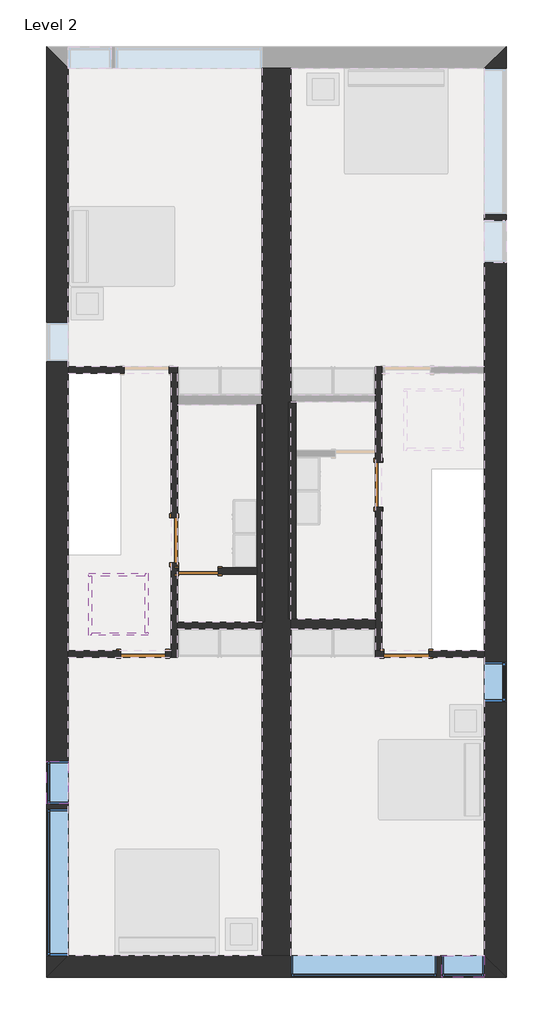
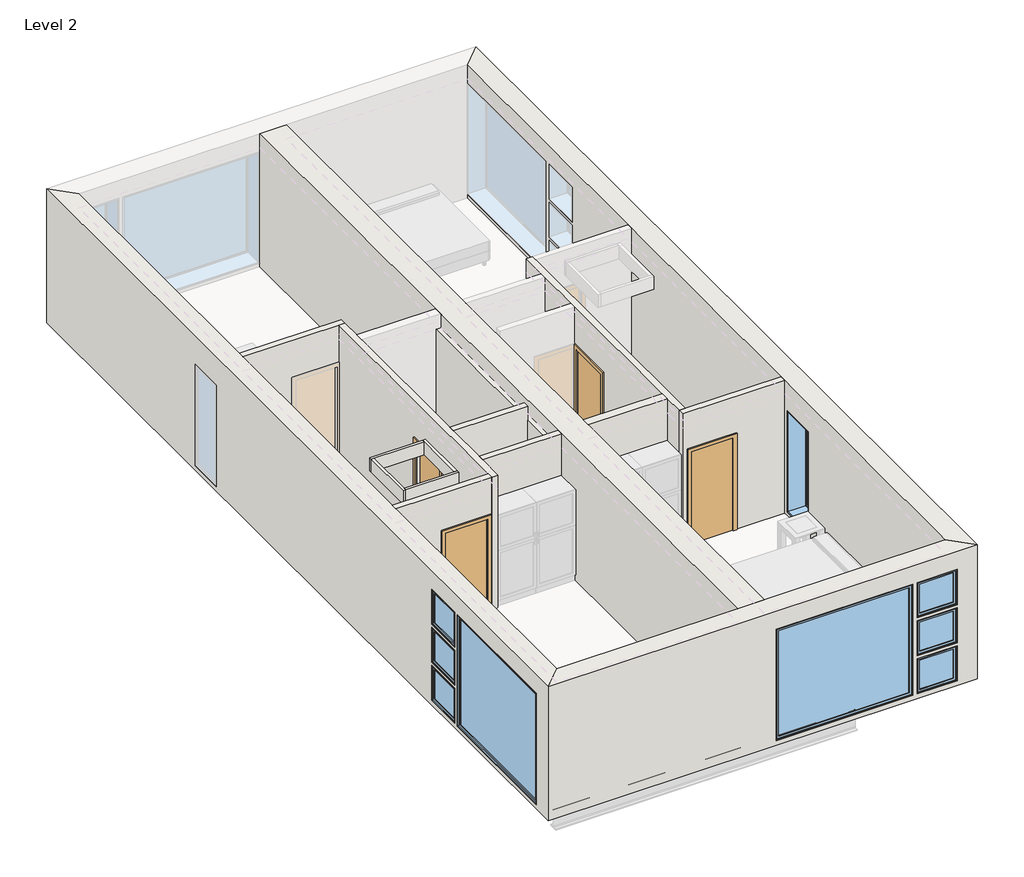
# One storey, part 1 of 2: 20 walls, 9 windows, 5 doors.
"""IFC4 building model written with IfcOpenShell, lengths in millimetres."""

import ifcopenshell
import ifcopenshell.guid

model = None  # the IFC model being written
_history = None  # IfcOwnerHistory: only IFC2X3 demands one
_inside = {}  # id of a spatial element -> (the spatial element, [elements in it])
_under = {}  # id of a project, library or spatial element -> (it, [spatial elements below it])
_declared = {}  # id of a project -> (the project, [libraries it declares])
_typed = {}  # id of a type object -> (the type object, [elements of that type])
_made_of = {}  # id of a material, layer set ... -> (it, [elements and type objects made of it])


def new_model(schema):
    """Start an empty IFC model of exactly this schema.

    Asked for "IFC4X3", IfcOpenShell would pick the latest addendum, in which some entities
    have other attributes; the version numbers below select the first issue.
    IFC2X3 requires an IfcOwnerHistory on every rooted entity: one is made here for all.
    """
    global model, _history
    if schema == "IFC4X3":
        model = ifcopenshell.file(schema_version=(4, 3, 0, 0))
    else:
        model = ifcopenshell.file(schema=schema)
    _inside.clear()
    _under.clear()
    _declared.clear()
    _typed.clear()
    _made_of.clear()
    _history = None
    if model.schema == "IFC2X3":
        org = make("IfcOrganization", Name="unknown")
        user = make(
            "IfcPersonAndOrganization",
            ThePerson=make("IfcPerson", FamilyName="unknown"),
            TheOrganization=org,
        )
        app = make(
            "IfcApplication",
            ApplicationDeveloper=org,
            Version="unknown",
            ApplicationFullName="unknown",
            ApplicationIdentifier="unknown",
        )
        _history = make(
            "IfcOwnerHistory",
            OwningUser=user,
            OwningApplication=app,
            ChangeAction="ADDED",
            CreationDate=0,
        )
    return model


def make(cls, **values):
    """One entity of the class cls with the attributes given. An attribute that is None is left unset."""
    return model.create_entity(
        cls, **{name: value for name, value in values.items() if value is not None}
    )


def rooted(cls, **values):
    """An entity with a GlobalId (a new one), such as an element, a storey or a relation."""
    return make(cls, GlobalId=ifcopenshell.guid.new(), OwnerHistory=_history, **values)


def si_unit(unit_type, name, prefix=None):
    """IfcSIUnit, for example si_unit("LENGTHUNIT", "METRE", prefix="MILLI")."""
    return make("IfcSIUnit", UnitType=unit_type, Prefix=prefix, Name=name)


def assignment(units):
    """IfcUnitAssignment: the units of a project."""
    return None if units is None else make("IfcUnitAssignment", Units=units)


def point(xyz):
    """IfcCartesianPoint."""
    return None if xyz is None else make("IfcCartesianPoint", Coordinates=xyz)


def direction(xyz):
    """IfcDirection."""
    return None if xyz is None else make("IfcDirection", DirectionRatios=xyz)


def frame(location, z_axis=None, x_axis=None):
    """IfcAxis2Placement3D, a coordinate frame: its origin and axes. An axis left out is left unset."""
    return make(
        "IfcAxis2Placement3D",
        Location=point(location),
        Axis=direction(z_axis),
        RefDirection=direction(x_axis),
    )


def origin():
    """The frame at (0, 0, 0) with its axes left unset."""
    return frame((0.0, 0.0, 0.0))


def origin_with_axes():
    """The frame at (0, 0, 0) with the z axis (0, 0, 1) and the x axis (1, 0, 0) written out."""
    return frame((0.0, 0.0, 0.0), z_axis=(0.0, 0.0, 1.0), x_axis=(1.0, 0.0, 0.0))


def place(relative_to, where):
    """IfcLocalPlacement: puts the frame where relative to a parent placement (None: the world)."""
    return make(
        "IfcLocalPlacement", PlacementRelTo=relative_to, RelativePlacement=where
    )


def context(
    kind, dimensions, precision=None, world=None, true_north=None, identifier=None
):
    """IfcGeometricRepresentationContext, for example the 3D "Model" context."""
    return make(
        "IfcGeometricRepresentationContext",
        ContextIdentifier=identifier,
        ContextType=kind,
        CoordinateSpaceDimension=dimensions,
        Precision=precision,
        WorldCoordinateSystem=world,
        TrueNorth=true_north,
    )


def project(units=None, contexts=None):
    """IfcProject with its units and contexts."""
    return rooted(
        "IfcProject",
        Name="project",
        RepresentationContexts=contexts,
        UnitsInContext=assignment(units),
    )


def spatial(cls, under=None, at=None, **own):
    """A site, building, storey or space (cls), placed at a placement, below another one or the project."""
    s = rooted(cls, ObjectPlacement=at, **own)
    if under is not None:
        _under.setdefault(under.id(), (under, []))[1].append(s)
    return s


def polyline(points):
    """IfcPolyline through the points."""
    return make("IfcPolyline", Points=[point(p) for p in points])


def outline(outer, holes=None, kind="AREA"):
    """IfcArbitraryClosedProfileDef: a profile drawn as a closed curve; with holes, ...WithVoids."""
    if holes is None:
        return make("IfcArbitraryClosedProfileDef", ProfileType=kind, OuterCurve=outer)
    return make(
        "IfcArbitraryProfileDefWithVoids",
        ProfileType=kind,
        OuterCurve=outer,
        InnerCurves=holes,
    )


def extrude(swept, where, along, depth):
    """IfcExtrudedAreaSolid: the profile swept, set in the frame where, extruded along a direction by depth."""
    return make(
        "IfcExtrudedAreaSolid",
        SweptArea=swept,
        Position=where,
        ExtrudedDirection=direction(along),
        Depth=depth,
    )


def faces_of(points, faces, orient=None, outer=None):
    """IfcFace entities. A face is a list of loops; a loop is a list of indices into points, from 0.

    orient and outer hold one flag for each loop. By default every Orientation is true, the
    first loop of a face is its IfcFaceOuterBound and the others are IfcFaceBound.
    """
    made = []
    for i, loops in enumerate(faces):
        bounds = []
        for j, loop in enumerate(loops):
            is_outer = j == 0 if outer is None else outer[i][j]
            bounds.append(
                make(
                    "IfcFaceOuterBound" if is_outer else "IfcFaceBound",
                    Bound=make("IfcPolyLoop", Polygon=[points[k] for k in loop]),
                    Orientation=True if orient is None else orient[i][j],
                )
            )
        made.append(make("IfcFace", Bounds=bounds))
    return made


def faceted_brep(points, faces, orient=None, outer=None, voids=None):
    """IfcFacetedBrep: a solid bounded by flat faces; with voids (closed shells), ...WithVoids."""
    shared = [point(p) for p in points]
    hull = make("IfcClosedShell", CfsFaces=faces_of(shared, faces, orient, outer))
    if voids is None:
        return make("IfcFacetedBrep", Outer=hull)
    return make(
        "IfcFacetedBrepWithVoids",
        Outer=hull,
        Voids=[
            make(cls, CfsFaces=faces_of(shared, fs, o, b)) for cls, fs, o, b in voids
        ],
    )


def shape(context_of_items, identifier, shape_type, items):
    """IfcShapeRepresentation: the items that make up one representation, for example the "Body"."""
    return make(
        "IfcShapeRepresentation",
        ContextOfItems=context_of_items,
        RepresentationIdentifier=identifier,
        RepresentationType=shape_type,
        Items=items,
    )


def source(mapping_origin, context_of_items, identifier, shape_type, items):
    """IfcRepresentationMap: a shape defined once, which mapped items show again and again."""
    return make(
        "IfcRepresentationMap",
        MappingOrigin=mapping_origin,
        MappedRepresentation=shape(context_of_items, identifier, shape_type, items),
    )


def transform(
    local_origin,
    x_axis=None,
    y_axis=None,
    z_axis=None,
    scale=None,
    scale2=None,
    scale3=None,
    uniform=True,
):
    """IfcCartesianTransformationOperator3D, or its non-uniform kind. x_axis, y_axis, z_axis: its Axis1, 2, 3."""
    if uniform:
        return make(
            "IfcCartesianTransformationOperator3D",
            Axis1=direction(x_axis),
            Axis2=direction(y_axis),
            LocalOrigin=point(local_origin),
            Scale=scale,
            Axis3=direction(z_axis),
        )
    return make(
        "IfcCartesianTransformationOperator3DnonUniform",
        Axis1=direction(x_axis),
        Axis2=direction(y_axis),
        LocalOrigin=point(local_origin),
        Scale=scale,
        Axis3=direction(z_axis),
        Scale2=scale2,
        Scale3=scale3,
    )


def mapped(mapping_source, mapping_target):
    """IfcMappedItem: shows the shape of a source again, moved by a transform."""
    return make(
        "IfcMappedItem", MappingSource=mapping_source, MappingTarget=mapping_target
    )


def made_of(thing, what):
    """Note that an element or type object is made of a material, layer set ...; save() writes the relation."""
    if what is not None:
        _made_of.setdefault(what.id(), (what, []))[1].append(thing)
    return thing


def element(
    cls,
    number,
    at=None,
    inside=None,
    cuts=None,
    type_object=None,
    material=None,
    context=None,
    identifier="Body",
    shape_type=None,
    held_by="IfcProductDefinitionShape",
    body=None,
    shapes=None,
    **own,
):
    """One element of the class cls, such as IfcWall. Its Tag is "e" and its number.

    at: its placement. inside: the storey or other place that contains it. cuts: it is an
    opening in that element (IfcRelVoidsElement). A single representation is given by context,
    identifier, shape_type and body (its items); several are given by shapes. held_by: the class
    of the entity that holds the representations. save() writes the other relations.
    """
    e = rooted(cls, Tag="e%d" % number, ObjectPlacement=at, **own)
    if body is not None:
        shapes = [shape(context, identifier, shape_type, body)]
    if shapes is not None:
        e.Representation = make(held_by, Representations=shapes)
    if inside is not None:
        _inside.setdefault(inside.id(), (inside, []))[1].append(e)
    if cuts is not None:
        rooted(
            "IfcRelVoidsElement", RelatingBuildingElement=cuts, RelatedOpeningElement=e
        )
    if type_object is not None:
        _typed.setdefault(type_object.id(), (type_object, []))[1].append(e)
    return made_of(e, material)


def aggregate(whole, parts):
    """IfcRelAggregates: a whole, such as a stair, and the parts it consists of."""
    return rooted("IfcRelAggregates", RelatingObject=whole, RelatedObjects=parts)


def save(model, path):
    """Write the relations noted so far, then the file.

    IfcRelAggregates (storeys below a building ...), IfcRelContainedInSpatialStructure (elements
    in a storey), IfcRelDefinesByType, IfcRelAssociatesMaterial and IfcRelDeclares: one each for
    every whole, place, type object, material and project.
    """
    for whole, parts in _under.values():
        aggregate(whole, parts)
    for where, things in _inside.values():
        rooted(
            "IfcRelContainedInSpatialStructure",
            RelatedElements=things,
            RelatingStructure=where,
        )
    for kind, things in _typed.values():
        rooted("IfcRelDefinesByType", RelatedObjects=things, RelatingType=kind)
    for what, things in _made_of.values():
        rooted("IfcRelAssociatesMaterial", RelatedObjects=things, RelatingMaterial=what)
    for by, libraries in _declared.values():
        rooted("IfcRelDeclares", RelatingContext=by, RelatedDefinitions=libraries)
    model.write(path)


def m_single_flush_0762_x_2032mm_e53dc8c7(model_context):
    return source(origin(), model_context, "Body", "SweptSolid", [
        extrude(outline(polyline([(2108.0, -457.0), (0.0, -457.0), (0.0, -381.0), (2032.0, -381.0), (2032.0, 381.0), (0.0, 381.0), (0.0, 457.0), (2108.0, 457.0), (2108.0, -457.0)])), frame((0.0, 62.0, 0.0), z_axis=(0.0, 1.0, 0.0), x_axis=(0.0, 0.0, 1.0)), (0.0, 0.0, 1.0), 25.0),
        extrude(outline(polyline([(2108.0, 457.0), (2108.0, -457.0), (0.0, -457.0), (0.0, -381.0), (2032.0, -381.0), (2032.0, 381.0), (0.0, 381.0), (0.0, 457.0), (2108.0, 457.0)])), frame((0.0, -87.0, 0.0), z_axis=(0.0, 1.0, 0.0), x_axis=(0.0, 0.0, 1.0)), (0.0, 0.0, 1.0), 25.0),
        extrude(outline(polyline([(381.0, 11.0), (-381.0, 11.0), (-381.0, 62.0), (381.0, 62.0), (381.0, 11.0)])), origin_with_axes(), (0.0, 0.0, 1.0), 2032.0),
    ])


def m_single_flush_0864_x_2032mm_f1a57c69(model_context):
    return source(origin(), model_context, "Body", "SweptSolid", [
        extrude(outline(polyline([(2108.0, -508.0), (0.0, -508.0), (0.0, -432.0), (2032.0, -432.0), (2032.0, 432.0), (0.0, 432.0), (0.0, 508.0), (2108.0, 508.0), (2108.0, -508.0)])), frame((0.0, 62.0, 0.0), z_axis=(0.0, 1.0, 0.0), x_axis=(0.0, 0.0, 1.0)), (0.0, 0.0, 1.0), 25.0),
        extrude(outline(polyline([(2108.0, 508.0), (2108.0, -508.0), (0.0, -508.0), (0.0, -432.0), (2032.0, -432.0), (2032.0, 432.0), (0.0, 432.0), (0.0, 508.0), (2108.0, 508.0)])), frame((0.0, -87.0, 0.0), z_axis=(0.0, 1.0, 0.0), x_axis=(0.0, 0.0, 1.0)), (0.0, 0.0, 1.0), 25.0),
        extrude(outline(polyline([(432.0, 11.0), (-432.0, 11.0), (-432.0, 62.0), (432.0, 62.0), (432.0, 11.0)])), origin_with_axes(), (0.0, 0.0, 1.0), 2032.0),
    ])


def m_single_flush_0864_x_2032mm_954ee019(model_context):
    return source(origin(), model_context, "Body", "SweptSolid", [
        extrude(outline(polyline([(2108.0, -508.0), (0.0, -508.0), (0.0, -432.0), (2032.0, -432.0), (2032.0, 432.0), (0.0, 432.0), (0.0, 508.0), (2108.0, 508.0), (2108.0, -508.0)])), frame((0.0, -87.0, 0.0), z_axis=(0.0, 1.0, 0.0), x_axis=(0.0, 0.0, 1.0)), (0.0, 0.0, 1.0), 25.0),
        extrude(outline(polyline([(2108.0, 508.0), (2108.0, -508.0), (0.0, -508.0), (0.0, -432.0), (2032.0, -432.0), (2032.0, 432.0), (0.0, 432.0), (0.0, 508.0), (2108.0, 508.0)])), frame((0.0, 62.0, 0.0), z_axis=(0.0, 1.0, 0.0), x_axis=(0.0, 0.0, 1.0)), (0.0, 0.0, 1.0), 25.0),
        extrude(outline(polyline([(432.0, -11.0), (432.0, -62.0), (-432.0, -62.0), (-432.0, -11.0), (432.0, -11.0)])), origin_with_axes(), (0.0, 0.0, 1.0), 2032.0),
    ])


def m_casement_819mm_x_759mm_6ad0bdaf(model_context):
    return source(origin(), model_context, "Body", "SweptSolid", [
        extrude(outline(polyline([(346.0, 160.925), (-346.0, 160.925), (-346.0, 173.625), (346.0, 173.625), (346.0, 160.925)])), frame((0.0, 0.0, 978.5), z_axis=(0.0, 0.0, 1.0), x_axis=(1.0, 0.0, 0.0)), (0.0, 0.0, 1.0), 632.0),
        extrude(outline(polyline([(1654.95, -390.45), (934.05, -390.45), (934.05, 390.45), (1654.95, 390.45), (1654.95, -390.45)]), holes=[polyline([(1610.5, -346.0), (1610.5, 346.0), (978.5, 346.0), (978.5, -346.0), (1610.5, -346.0)])]), frame((0.0, 145.05, 0.0), z_axis=(0.0, 1.0, 0.0), x_axis=(0.0, 0.0, 1.0)), (0.0, 0.0, 1.0), 44.45),
        extrude(outline(polyline([(1674.0, -409.5), (915.0, -409.5), (915.0, 409.5), (1674.0, 409.5), (1674.0, -409.5)]), holes=[polyline([(1642.25, -377.75), (1642.25, 377.75), (946.75, 377.75), (946.75, -377.75), (1642.25, -377.75)])]), frame((0.0, -208.5, 0.0), z_axis=(0.0, 1.0, 0.0), x_axis=(0.0, 0.0, 1.0)), (0.0, 0.0, 1.0), 353.55),
        extrude(outline(polyline([(1674.0, 409.5), (1674.0, -409.5), (915.0, -409.5), (915.0, 409.5), (1674.0, 409.5)]), holes=[polyline([(1654.95, 390.45), (934.05, 390.45), (934.05, -390.45), (1654.95, -390.45), (1654.95, 390.45)])]), frame((0.0, 145.05, 0.0), z_axis=(0.0, 1.0, 0.0), x_axis=(0.0, 0.0, 1.0)), (0.0, 0.0, 1.0), 63.45),
    ])


def m_fixed_2800mm_x_2410mm_0fa4d817(model_context):
    return source(origin(), model_context, "Body", "SweptSolid", [
        extrude(outline(polyline([(-1337.0, 186.5), (1337.0, 186.5), (1337.0, 174.5), (-1337.0, 174.5), (-1337.0, 186.5)])), frame((0.0, 0.0, 163.0), z_axis=(0.0, 0.0, 1.0), x_axis=(1.0, 0.0, 0.0)), (0.0, 0.0, 1.0), 2284.0),
        extrude(outline(polyline([(2491.0, -1381.0), (119.0, -1381.0), (119.0, 1381.0), (2491.0, 1381.0), (2491.0, -1381.0)]), holes=[polyline([(2447.0, -1337.0), (2447.0, 1337.0), (163.0, 1337.0), (163.0, -1337.0), (2447.0, -1337.0)])]), frame((0.0, 158.5, 0.0), z_axis=(0.0, 1.0, 0.0), x_axis=(0.0, 0.0, 1.0)), (0.0, 0.0, 1.0), 44.0),
        extrude(outline(polyline([(2510.0, -1400.0), (100.0, -1400.0), (100.0, 1400.0), (2510.0, 1400.0), (2510.0, -1400.0)]), holes=[polyline([(2491.0, -1381.0), (2491.0, 1381.0), (119.0, 1381.0), (119.0, -1381.0), (2491.0, -1381.0)])]), frame((0.0, 158.5, 0.0), z_axis=(0.0, 1.0, 0.0), x_axis=(0.0, 0.0, 1.0)), (0.0, 0.0, 1.0), 63.0),
        extrude(outline(polyline([(2510.0, -1400.0), (100.0, -1400.0), (100.0, 1400.0), (2510.0, 1400.0), (2510.0, -1400.0)]), holes=[polyline([(2478.0, -1368.0), (2478.0, 1368.0), (132.0, 1368.0), (132.0, -1368.0), (2478.0, -1368.0)])]), frame((0.0, -195.5, 0.0), z_axis=(0.0, 1.0, 0.0), x_axis=(0.0, 0.0, 1.0)), (0.0, 0.0, 1.0), 354.0),
    ])


def m_fixed_750mm_x_2200mm_8ca0da28(model_context):
    return source(origin(), model_context, "Body", "SweptSolid", [
        extrude(outline(polyline([(-312.0, 186.5), (312.0, 186.5), (312.0, 174.5), (-312.0, 174.5), (-312.0, 186.5)])), frame((0.0, 0.0, 163.0), z_axis=(0.0, 0.0, 1.0), x_axis=(1.0, 0.0, 0.0)), (0.0, 0.0, 1.0), 2074.0),
        extrude(outline(polyline([(2281.0, -356.0), (119.0, -356.0), (119.0, 356.0), (2281.0, 356.0), (2281.0, -356.0)]), holes=[polyline([(2237.0, -312.0), (2237.0, 312.0), (163.0, 312.0), (163.0, -312.0), (2237.0, -312.0)])]), frame((0.0, 158.5, 0.0), z_axis=(0.0, 1.0, 0.0), x_axis=(0.0, 0.0, 1.0)), (0.0, 0.0, 1.0), 44.0),
        extrude(outline(polyline([(2300.0, -375.0), (100.0, -375.0), (100.0, 375.0), (2300.0, 375.0), (2300.0, -375.0)]), holes=[polyline([(2281.0, -356.0), (2281.0, 356.0), (119.0, 356.0), (119.0, -356.0), (2281.0, -356.0)])]), frame((0.0, 158.5, 0.0), z_axis=(0.0, 1.0, 0.0), x_axis=(0.0, 0.0, 1.0)), (0.0, 0.0, 1.0), 63.0),
        extrude(outline(polyline([(2300.0, -375.0), (100.0, -375.0), (100.0, 375.0), (2300.0, 375.0), (2300.0, -375.0)]), holes=[polyline([(2268.0, -343.0), (2268.0, 343.0), (132.0, 343.0), (132.0, -343.0), (2268.0, -343.0)])]), frame((0.0, -195.5, 0.0), z_axis=(0.0, 1.0, 0.0), x_axis=(0.0, 0.0, 1.0)), (0.0, 0.0, 1.0), 354.0),
    ])


def m_fixed_819mm_x_759mm_7938e442(model_context):
    return source(origin(), model_context, "Body", "SweptSolid", [
        extrude(outline(polyline([(-346.5, 186.5), (346.5, 186.5), (346.5, 174.5), (-346.5, 174.5), (-346.5, 186.5)])), frame((0.0, 0.0, 163.0), z_axis=(0.0, 0.0, 1.0), x_axis=(1.0, 0.0, 0.0)), (0.0, 0.0, 1.0), 633.0),
        extrude(outline(polyline([(840.0, -390.5), (119.0, -390.5), (119.0, 390.5), (840.0, 390.5), (840.0, -390.5)]), holes=[polyline([(796.0, -346.5), (796.0, 346.5), (163.0, 346.5), (163.0, -346.5), (796.0, -346.5)])]), frame((0.0, 158.5, 0.0), z_axis=(0.0, 1.0, 0.0), x_axis=(0.0, 0.0, 1.0)), (0.0, 0.0, 1.0), 44.0),
        extrude(outline(polyline([(859.0, -409.5), (100.0, -409.5), (100.0, 409.5), (859.0, 409.5), (859.0, -409.5)]), holes=[polyline([(840.0, -390.5), (840.0, 390.5), (119.0, 390.5), (119.0, -390.5), (840.0, -390.5)])]), frame((0.0, 158.5, 0.0), z_axis=(0.0, 1.0, 0.0), x_axis=(0.0, 0.0, 1.0)), (0.0, 0.0, 1.0), 63.0),
        extrude(outline(polyline([(859.0, -409.5), (100.0, -409.5), (100.0, 409.5), (859.0, 409.5), (859.0, -409.5)]), holes=[polyline([(827.0, -377.5), (827.0, 377.5), (132.0, 377.5), (132.0, -377.5), (827.0, -377.5)])]), frame((0.0, -195.5, 0.0), z_axis=(0.0, 1.0, 0.0), x_axis=(0.0, 0.0, 1.0)), (0.0, 0.0, 1.0), 354.0),
    ])


model = new_model("IFC4")

# Units and contexts
model_context = context("Model", 3, world=origin())
ifc_project = project(units=[si_unit("LENGTHUNIT", "METRE", prefix="MILLI")], contexts=[model_context])

# Site, building, storey
site = spatial("IfcSite", under=ifc_project)
building = spatial("IfcBuilding", under=site)
storey = spatial("IfcBuildingStorey", under=building, Name="Level 2", Elevation=3100.0)

# Doors
placement = place(None, origin())
m_single_flush_0762_x_2032mm_shape = m_single_flush_0762_x_2032mm_e53dc8c7(model_context)
element("IfcDoor", 1, ObjectType="M_Single-Flush : 0762 x 2032mm", at=placement, inside=storey, context=model_context, shape_type="MappedRepresentation", body=[
    mapped(m_single_flush_0762_x_2032mm_shape, transform((2907.0, -10032.0511785, 3100.0), x_axis=(-1.0, 0.0, 0.0), y_axis=(0.0, -1.0, 0.0), z_axis=(0.0, 0.0, 1.0))),
])
m_single_flush_0864_x_2032mm_shape = m_single_flush_0864_x_2032mm_f1a57c69(model_context)
element("IfcDoor", 2, ObjectType="M_Single-Flush : 0864 x 2032mm", at=placement, inside=storey, context=model_context, shape_type="MappedRepresentation", body=[
    mapped(m_single_flush_0864_x_2032mm_shape, transform((6889.3, -11612.0, 3100.0), x_axis=(-1.0, 0.0, 0.0), y_axis=(0.0, -1.0, 0.0), z_axis=(0.0, 0.0, 1.0))),
])
element("IfcDoor", 3, ObjectType="M_Single-Flush : 0864 x 2032mm", at=placement, inside=storey, context=model_context, shape_type="MappedRepresentation", body=[
    mapped(m_single_flush_0864_x_2032mm_shape, transform((2444.0, -9438.0511785, 3100.0), x_axis=(0.0, -1.0, 0.0), y_axis=(1.0, 0.0, 0.0), z_axis=(0.0, 0.0, 1.0))),
])
element("IfcDoor", 4, ObjectType="M_Single-Flush : 0864 x 2032mm", at=placement, inside=storey, context=model_context, shape_type="MappedRepresentation", body=[
    mapped(m_single_flush_0864_x_2032mm_shape, transform((6356.0, -8377.3842351, 3100.0), x_axis=(0.0, 1.0, 0.0), y_axis=(-1.0, 0.0, 0.0), z_axis=(0.0, 0.0, 1.0))),
])
m_single_flush_0864_x_2032mm_2_shape = m_single_flush_0864_x_2032mm_954ee019(model_context)
element("IfcDoor", 5, ObjectType="M_Single-Flush : 0864 x 2032mm", at=placement, inside=storey, context=model_context, shape_type="MappedRepresentation", body=[
    mapped(m_single_flush_0864_x_2032mm_2_shape, transform((1850.0, -11612.0, 3100.0), x_axis=(1.0, 0.0, 0.0), y_axis=(0.0, 1.0, 0.0), z_axis=(0.0, 0.0, 1.0))),
])

# Walls
element("IfcWall", 6, ObjectType="Party Wall - CMU Residential Unit Dimising Wall", at=placement, inside=storey, context=model_context, shape_type="Brep", body=[
    faceted_brep([(4125.0, -17383.0, 6000.0), (4125.0, -11134.0, 6000.0), (4125.0, -11010.0, 6000.0), (4125.0, -6850.0, 6000.0), (4125.0, -6666.0, 6000.0), (4125.0, -417.0, 6000.0), (4125.0, -417.0, 5610.0), (4125.0, -417.0, 3200.0), (4125.0, -417.0, 3100.0), (4125.0, -6666.0, 3100.0), (4125.0, -6850.0, 3100.0), (4125.0, -6850.0, 5695.0), (4125.0, -11010.0, 5695.0), (4125.0, -11010.0, 3100.0), (4125.0, -11134.0, 3100.0), (4125.0, -17383.0, 3100.0), (4675.0, -417.0, 6000.0), (4675.0, -6666.0, 6000.0), (4675.0, -6790.0, 6000.0), (4675.0, -10950.0, 6000.0), (4675.0, -11134.0, 6000.0), (4675.0, -17383.0, 6000.0), (4675.0, -17383.0, 5610.0), (4675.0, -17383.0, 3200.0), (4675.0, -17383.0, 3100.0), (4675.0, -11134.0, 3100.0), (4675.0, -10950.0, 3100.0), (4675.0, -10950.0, 5695.0), (4675.0, -6790.0, 5695.0), (4675.0, -6790.0, 3100.0), (4675.0, -6666.0, 3100.0), (4675.0, -417.0, 3100.0), (4618.0, -6790.0, 3100.0), (4618.0, -10950.0, 3100.0), (4182.0, -11010.0, 3100.0), (4182.0, -6850.0, 3100.0), (4618.0, -10950.0, 5695.0), (4618.0, -6790.0, 5695.0), (4182.0, -6850.0, 5695.0), (4182.0, -11010.0, 5695.0)], [[[0, 1, 2, 3, 4, 5, 6, 7, 8, 9, 10, 11, 12, 13, 14, 15]], [[16, 17, 18, 19, 20, 21, 22, 23, 24, 25, 26, 27, 28, 29, 30, 31]], [[8, 31, 30, 29, 32, 33, 26, 25, 24, 15, 14, 13, 34, 35, 10, 9]], [[5, 4, 3, 2, 1, 0, 21, 20, 19, 18, 17, 16]], [[8, 7, 6, 5, 16, 31]], [[0, 15, 24, 23, 22, 21]], [[36, 33, 32, 37]], [[36, 37, 28, 27]], [[37, 32, 29, 28]], [[33, 36, 27, 26]], [[38, 35, 34, 39]], [[38, 39, 12, 11]], [[35, 38, 11, 10]], [[39, 34, 13, 12]]]),
])
element("IfcWall", 7, ObjectType="Exterior - Brick on Block", at=placement, inside=storey, context=model_context, shape_type="Brep", body=[
    faceted_brep([(8383.0, -417.0, 3100.0), (8383.0, -6126.0, 3100.0), (8383.0, -6250.0, 3100.0), (8383.0, -17383.0, 3100.0), (8383.0, -17383.0, 3200.0), (8383.0, -17383.0, 3959.0), (8383.0, -17383.0, 4025.5), (8383.0, -17383.0, 4784.5), (8383.0, -17383.0, 4851.0), (8383.0, -17383.0, 5610.0), (8383.0, -17383.0, 6000.0), (8383.0, -11674.0, 6000.0), (8383.0, -11550.0, 6000.0), (8383.0, -6250.0, 6000.0), (8383.0, -6126.0, 6000.0), (8383.0, -417.0, 6000.0), (8383.0, -417.0, 5610.0), (8383.0, -3217.0, 5610.0), (8383.0, -3217.0, 3200.0), (8383.0, -417.0, 3200.0), (8383.0, -3317.0, 4851.0), (8383.0, -3317.0, 5610.0), (8383.0, -4136.0, 5610.0), (8383.0, -4136.0, 4851.0), (8383.0, -4136.0, 4784.5), (8383.0, -4136.0, 4025.5), (8383.0, -3317.0, 4025.5), (8383.0, -3317.0, 4784.5), (8383.0, -3317.0, 3200.0), (8383.0, -3317.0, 3959.0), (8383.0, -4136.0, 3959.0), (8383.0, -4136.0, 3200.0), (8383.0, -11774.0, 3200.0), (8383.0, -11774.0, 5400.0), (8383.0, -12524.0, 5400.0), (8383.0, -12524.0, 3200.0), (8800.0, -17800.0, 3100.0), (8800.0, 0.0, 3100.0), (8800.0, 0.0, 6000.0), (8800.0, -17800.0, 6000.0), (8800.0, -417.0, 5610.0), (8800.0, -417.0, 3200.0), (8800.0, -3217.0, 3200.0), (8800.0, -3217.0, 5610.0), (8800.0, -3317.0, 5610.0), (8800.0, -3317.0, 4851.0), (8800.0, -4136.0, 4851.0), (8800.0, -4136.0, 5610.0), (8800.0, -4136.0, 4025.5), (8800.0, -4136.0, 4784.5), (8800.0, -3317.0, 4784.5), (8800.0, -3317.0, 4025.5), (8800.0, -3317.0, 3959.0), (8800.0, -3317.0, 3200.0), (8800.0, -4136.0, 3200.0), (8800.0, -4136.0, 3959.0), (8800.0, -11774.0, 5400.0), (8800.0, -11774.0, 3200.0), (8800.0, -12524.0, 3200.0), (8800.0, -12524.0, 5400.0)], [[[0, 1, 2, 3, 4, 5, 6, 7, 8, 9, 10, 11, 12, 13, 14, 15, 16, 17, 18, 19], [20, 21, 22, 23], [24, 25, 26, 27], [28, 29, 30, 31], [32, 33, 34, 35]], [[36, 37, 38, 39], [40, 41, 42, 43], [44, 45, 46, 47], [48, 49, 50, 51], [52, 53, 54, 55], [56, 57, 58, 59]], [[3, 2, 1, 0, 37, 36]], [[15, 14, 13, 12, 11, 10, 39, 38]], [[15, 38, 37, 0, 19, 16]], [[10, 9, 8, 7, 6, 5, 4, 3, 36, 39]], [[19, 41, 40, 16]], [[42, 18, 17, 43]], [[41, 19, 18, 42]], [[16, 40, 43, 17]], [[21, 20, 45, 44]], [[22, 21, 44, 47]], [[23, 22, 47, 46]], [[20, 23, 46, 45]], [[48, 25, 24, 49]], [[51, 26, 25, 48]], [[26, 51, 50, 27]], [[49, 24, 27, 50]], [[29, 28, 53, 52]], [[30, 29, 52, 55]], [[31, 30, 55, 54]], [[28, 31, 54, 53]], [[32, 57, 56, 33]], [[34, 59, 58, 35]], [[57, 32, 35, 58]], [[59, 34, 33, 56]]]),
])
element("IfcWall", 8, ObjectType="Exterior - Brick on Block", at=placement, inside=storey, context=model_context, shape_type="Brep", body=[
    faceted_brep([(8383.0, -17383.0, 3100.0), (4675.0, -17383.0, 3100.0), (4125.0, -17383.0, 3100.0), (417.0, -17383.0, 3100.0), (417.0, -17383.0, 3200.0), (417.0, -17383.0, 5610.0), (417.0, -17383.0, 6000.0), (4125.0, -17383.0, 6000.0), (4675.0, -17383.0, 6000.0), (8383.0, -17383.0, 6000.0), (8383.0, -17383.0, 5610.0), (7564.0, -17383.0, 5610.0), (7564.0, -17383.0, 4851.0), (8383.0, -17383.0, 4851.0), (8383.0, -17383.0, 4784.5), (7564.0, -17383.0, 4784.5), (7564.0, -17383.0, 4025.5), (8383.0, -17383.0, 4025.5), (8383.0, -17383.0, 3959.0), (7564.0, -17383.0, 3959.0), (7564.0, -17383.0, 3200.0), (8383.0, -17383.0, 3200.0), (7475.0, -17383.0, 3200.0), (7475.0, -17383.0, 5610.0), (4675.0, -17383.0, 5610.0), (4675.0, -17383.0, 3200.0), (0.0, -17800.0, 3100.0), (8800.0, -17800.0, 3100.0), (8800.0, -17800.0, 6000.0), (0.0, -17800.0, 6000.0), (7475.0, -17800.0, 3200.0), (4675.0, -17800.0, 3200.0), (4675.0, -17800.0, 5610.0), (7475.0, -17800.0, 5610.0), (8383.0, -17800.0, 5610.0), (8383.0, -17800.0, 4851.0), (7564.0, -17800.0, 4851.0), (7564.0, -17800.0, 5610.0), (7564.0, -17800.0, 4025.5), (7564.0, -17800.0, 4784.5), (8383.0, -17800.0, 4784.5), (8383.0, -17800.0, 4025.5), (8383.0, -17800.0, 3959.0), (8383.0, -17800.0, 3200.0), (7564.0, -17800.0, 3200.0), (7564.0, -17800.0, 3959.0)], [[[0, 1, 2, 3, 4, 5, 6, 7, 8, 9, 10, 11, 12, 13, 14, 15, 16, 17, 18, 19, 20, 21], [22, 23, 24, 25]], [[26, 27, 28, 29], [30, 31, 32, 33], [34, 35, 36, 37], [38, 39, 40, 41], [42, 43, 44, 45]], [[3, 2, 1, 0, 27, 26]], [[9, 8, 7, 6, 29, 28]], [[9, 28, 27, 0, 21, 18, 17, 14, 13, 10]], [[6, 5, 4, 3, 26, 29]], [[23, 22, 30, 33]], [[24, 23, 33, 32]], [[25, 24, 32, 31]], [[22, 25, 31, 30]], [[13, 35, 34, 10]], [[10, 34, 37, 11]], [[11, 37, 36, 12]], [[35, 13, 12, 36]], [[15, 39, 38, 16]], [[16, 38, 41, 17]], [[17, 41, 40, 14]], [[39, 15, 14, 40]], [[21, 43, 42, 18]], [[18, 42, 45, 19]], [[19, 45, 44, 20]], [[43, 21, 20, 44]]]),
])
element("IfcWall", 9, ObjectType="Exterior - Brick on Block", at=placement, inside=storey, context=model_context, shape_type="Brep", body=[
    faceted_brep([(417.0, -17383.0, 3100.0), (417.0, -11674.0, 3100.0), (417.0, -11550.0, 3100.0), (417.0, -417.0, 3100.0), (417.0, -417.0, 3200.0), (417.0, -417.0, 3959.0), (417.0, -417.0, 4025.5), (417.0, -417.0, 4784.5), (417.0, -417.0, 4851.0), (417.0, -417.0, 5610.0), (417.0, -417.0, 6000.0), (417.0, -6126.0, 6000.0), (417.0, -6250.0, 6000.0), (417.0, -11550.0, 6000.0), (417.0, -11674.0, 6000.0), (417.0, -17383.0, 6000.0), (417.0, -17383.0, 5610.0), (417.0, -14583.0, 5610.0), (417.0, -14583.0, 3200.0), (417.0, -17383.0, 3200.0), (417.0, -14483.0, 4851.0), (417.0, -14483.0, 5610.0), (417.0, -13664.0, 5610.0), (417.0, -13664.0, 4851.0), (417.0, -14483.0, 3200.0), (417.0, -14483.0, 3959.0), (417.0, -13664.0, 3959.0), (417.0, -13664.0, 3200.0), (417.0, -13664.0, 4784.5), (417.0, -13664.0, 4025.5), (417.0, -14483.0, 4025.5), (417.0, -14483.0, 4784.5), (417.0, -6026.0, 3200.0), (417.0, -6026.0, 5400.0), (417.0, -5276.0, 5400.0), (417.0, -5276.0, 3200.0), (0.0, 0.0, 3100.0), (0.0, -17800.0, 3100.0), (0.0, -17800.0, 6000.0), (0.0, 0.0, 6000.0), (0.0, -17383.0, 5610.0), (0.0, -17383.0, 3200.0), (0.0, -14583.0, 3200.0), (0.0, -14583.0, 5610.0), (0.0, -14483.0, 5610.0), (0.0, -14483.0, 4851.0), (0.0, -13664.0, 4851.0), (0.0, -13664.0, 5610.0), (0.0, -14483.0, 3959.0), (0.0, -14483.0, 3200.0), (0.0, -13664.0, 3200.0), (0.0, -13664.0, 3959.0), (0.0, -13664.0, 4025.5), (0.0, -13664.0, 4784.5), (0.0, -14483.0, 4784.5), (0.0, -14483.0, 4025.5), (0.0, -6026.0, 5400.0), (0.0, -6026.0, 3200.0), (0.0, -5276.0, 3200.0), (0.0, -5276.0, 5400.0)], [[[0, 1, 2, 3, 4, 5, 6, 7, 8, 9, 10, 11, 12, 13, 14, 15, 16, 17, 18, 19], [20, 21, 22, 23], [24, 25, 26, 27], [28, 29, 30, 31], [32, 33, 34, 35]], [[36, 37, 38, 39], [40, 41, 42, 43], [44, 45, 46, 47], [48, 49, 50, 51], [52, 53, 54, 55], [56, 57, 58, 59]], [[3, 2, 1, 0, 37, 36]], [[15, 14, 13, 12, 11, 10, 39, 38]], [[10, 9, 8, 7, 6, 5, 4, 3, 36, 39]], [[15, 38, 37, 0, 19, 16]], [[19, 41, 40, 16]], [[42, 18, 17, 43]], [[41, 19, 18, 42]], [[16, 40, 43, 17]], [[21, 20, 45, 44]], [[22, 21, 44, 47]], [[23, 22, 47, 46]], [[20, 23, 46, 45]], [[25, 24, 49, 48]], [[26, 25, 48, 51]], [[27, 26, 51, 50]], [[24, 27, 50, 49]], [[29, 28, 53, 52]], [[30, 29, 52, 55]], [[31, 30, 55, 54]], [[28, 31, 54, 53]], [[32, 57, 56, 33]], [[34, 59, 58, 35]], [[57, 32, 35, 58]], [[59, 34, 33, 56]]]),
])
element("IfcWall", 10, ObjectType="Interior - Furring (152 mm Stud)", at=placement, inside=storey, context=model_context, shape_type="Brep", body=[
    faceted_brep([(4618.0, -6790.0, 3100.0), (4618.0, -10950.0, 3100.0), (4618.0, -10950.0, 5695.0), (4618.0, -6790.0, 5695.0), (4770.0, -6790.0, 3100.0), (4770.0, -6790.0, 5695.0), (4770.0, -10950.0, 5695.0), (4770.0, -10950.0, 3100.0), (4770.0, -7845.3842351, 3100.0), (4770.0, -7721.3842351, 3100.0), (4675.0, -6790.0, 3100.0), (4675.0, -10950.0, 3100.0), (4675.0, -10950.0, 5695.0), (4675.0, -6790.0, 5695.0)], [[[0, 1, 2, 3]], [[4, 5, 6, 7, 8, 9]], [[1, 0, 10, 4, 9, 8, 7, 11]], [[3, 2, 12, 6, 5, 13]], [[0, 3, 13, 5, 4, 10]], [[2, 1, 11, 7, 6, 12]]]),
])
element("IfcWall", 11, ObjectType="Interior - Furring (152 mm Stud)", at=placement, inside=storey, context=model_context, shape_type="Brep", body=[
    faceted_brep([(4182.0, -11010.0, 3100.0), (4182.0, -6850.0, 3100.0), (4182.0, -6850.0, 5695.0), (4182.0, -11010.0, 5695.0), (4030.0, -11010.0, 3100.0), (4030.0, -11010.0, 5695.0), (4030.0, -6850.0, 5695.0), (4030.0, -6850.0, 3100.0), (4030.0, -9970.0511785, 3100.0), (4030.0, -10094.0511785, 3100.0), (4125.0, -11010.0, 3100.0), (4125.0, -6850.0, 3100.0), (4125.0, -6850.0, 5695.0), (4125.0, -11010.0, 5695.0)], [[[0, 1, 2, 3]], [[4, 5, 6, 7, 8, 9]], [[1, 0, 10, 4, 9, 8, 7, 11]], [[3, 2, 12, 6, 5, 13]], [[2, 1, 11, 7, 6, 12]], [[0, 3, 13, 5, 4, 10]]]),
])
element("IfcWall", 12, ObjectType="Interior - Furring (38 mm Stud)", at=placement, inside=storey, context=model_context, shape_type="Brep", body=[
    faceted_brep([(807.45, -10124.45, 5712.0), (861.45, -10124.45, 5712.0), (1890.55, -10124.45, 5712.0), (1890.55, -10124.45, 6000.0), (861.45, -10124.45, 6000.0), (807.45, -10124.45, 6000.0), (807.45, -10070.45, 5712.0), (807.45, -10070.45, 6000.0), (1890.55, -10070.45, 6000.0), (1890.55, -10070.45, 5712.0)], [[[0, 1, 2, 3, 4, 5]], [[6, 7, 8, 9]], [[2, 1, 0, 6, 9]], [[5, 4, 3, 8, 7]], [[0, 5, 7, 6]], [[3, 2, 9, 8]]]),
])
element("IfcWall", 13, ObjectType="Interior - Furring (38 mm Stud)", at=placement, inside=storey, context=model_context, shape_type="Brep", body=[
    faceted_brep([(861.45, -11259.55, 5712.0), (861.45, -11205.55, 5712.0), (861.45, -10124.45, 5712.0), (861.45, -10124.45, 6000.0), (861.45, -11205.55, 6000.0), (861.45, -11259.55, 6000.0), (807.45, -11259.55, 5712.0), (807.45, -11259.55, 6000.0), (807.45, -10124.45, 6000.0), (807.45, -10124.45, 5712.0)], [[[0, 1, 2, 3, 4, 5]], [[6, 7, 8, 9]], [[2, 1, 0, 6, 9]], [[5, 4, 3, 8, 7]], [[0, 5, 7, 6]], [[3, 2, 9, 8]]]),
])
element("IfcWall", 14, ObjectType="Interior - Furring (38 mm Stud)", at=placement, inside=storey, context=model_context, shape_type="Brep", body=[
    faceted_brep([(1944.55, -11205.55, 5712.0), (1890.55, -11205.55, 5712.0), (861.45, -11205.55, 5712.0), (861.45, -11205.55, 6000.0), (1890.55, -11205.55, 6000.0), (1944.55, -11205.55, 6000.0), (1944.55, -11259.55, 5712.0), (1944.55, -11259.55, 6000.0), (861.45, -11259.55, 6000.0), (861.45, -11259.55, 5712.0)], [[[0, 1, 2, 3, 4, 5]], [[6, 7, 8, 9]], [[2, 1, 0, 6, 9]], [[5, 4, 3, 8, 7]], [[0, 5, 7, 6]], [[3, 2, 9, 8]]]),
])
element("IfcWall", 15, ObjectType="Interior - Furring (38 mm Stud)", at=placement, inside=storey, context=model_context, shape_type="Brep", body=[
    faceted_brep([(1890.55, -10070.45, 5712.0), (1890.55, -10124.45, 5712.0), (1890.55, -11205.55, 5712.0), (1890.55, -11205.55, 6000.0), (1890.55, -10124.45, 6000.0), (1890.55, -10070.45, 6000.0), (1944.55, -10070.45, 5712.0), (1944.55, -10070.45, 6000.0), (1944.55, -11205.55, 6000.0), (1944.55, -11205.55, 5712.0)], [[[0, 1, 2, 3, 4, 5]], [[6, 7, 8, 9]], [[2, 1, 0, 6, 9]], [[5, 4, 3, 8, 7]], [[0, 5, 7, 6]], [[3, 2, 9, 8]]]),
])
element("IfcWall", 16, ObjectType="Interior - Partition (92mm Stud)", at=placement, inside=storey, context=model_context, shape_type="Brep", body=[
    faceted_brep([(417.0, -6250.0, 6000.0), (417.0, -6250.0, 2612.0), (1431.4, -6250.0, 2612.0), (1555.4, -6250.0, 2612.0), (2506.0, -6250.0, 2612.0), (2506.0, -6250.0, 3100.0), (2506.0, -6250.0, 6000.0), (2382.0, -6250.0, 6000.0), (1483.3, -6250.0, 3100.0), (1483.3, -6250.0, 5132.0), (2347.3, -6250.0, 5132.0), (2347.3, -6250.0, 3100.0), (1555.4, -6250.0, 3100.0), (417.0, -6126.0, 2612.0), (417.0, -6126.0, 6000.0), (2506.0, -6126.0, 6000.0), (2506.0, -6126.0, 2612.0), (1483.3, -6126.0, 3100.0), (2347.3, -6126.0, 3100.0), (2347.3, -6126.0, 5132.0), (1483.3, -6126.0, 5132.0)], [[[0, 1, 2, 3, 4, 5, 6, 7], [8, 9, 10, 11, 12]], [[13, 14, 15, 16], [17, 18, 19, 20]], [[4, 3, 2, 1, 13, 16]], [[0, 7, 6, 15, 14]], [[6, 5, 4, 16, 15]], [[18, 17, 8, 12, 11]], [[19, 18, 11, 10]], [[20, 19, 10, 9]], [[17, 20, 9, 8]], [[0, 14, 13, 1]]]),
])
element("IfcWall", 17, ObjectType="Interior - Partition (92mm Stud)", at=placement, inside=storey, context=model_context, shape_type="Brep", body=[
    faceted_brep([(2382.0, -9870.0511785, 5132.0), (2382.0, -9870.0511785, 3100.0), (2382.0, -11550.0, 3100.0), (2382.0, -11674.0, 3100.0), (2382.0, -11674.0, 6000.0), (2382.0, -11550.0, 6000.0), (2382.0, -6250.0, 6000.0), (2382.0, -6250.0, 3100.0), (2382.0, -9006.0511785, 3100.0), (2382.0, -9006.0511785, 5132.0), (2506.0, -11674.0, 3100.0), (2506.0, -11134.0, 3100.0), (2506.0, -11010.0, 3100.0), (2506.0, -10094.0511785, 3100.0), (2506.0, -9970.0511785, 3100.0), (2506.0, -9870.0511785, 3100.0), (2506.0, -9870.0511785, 5132.0), (2506.0, -9006.0511785, 5132.0), (2506.0, -9006.0511785, 3100.0), (2506.0, -6850.0, 3100.0), (2506.0, -6666.0, 3100.0), (2506.0, -6250.0, 3100.0), (2506.0, -6250.0, 6000.0), (2506.0, -6666.0, 6000.0), (2506.0, -6850.0, 6000.0), (2506.0, -9970.0511785, 6000.0), (2506.0, -10094.0511785, 6000.0), (2506.0, -11010.0, 6000.0), (2506.0, -11134.0, 6000.0), (2506.0, -11674.0, 6000.0)], [[[0, 1, 2, 3, 4, 5, 6, 7, 8, 9]], [[10, 11, 12, 13, 14, 15, 16, 17, 18, 19, 20, 21, 22, 23, 24, 25, 26, 27, 28, 29]], [[8, 7, 21, 20, 19, 18]], [[3, 2, 1, 15, 14, 13, 12, 11, 10]], [[6, 5, 4, 29, 28, 27, 26, 25, 24, 23, 22]], [[7, 6, 22, 21]], [[4, 3, 10, 29]], [[16, 15, 1, 0]], [[17, 16, 0, 9]], [[18, 17, 9, 8]]]),
])
element("IfcWall", 18, ObjectType="Interior - Partition (92mm Stud)", at=placement, inside=storey, context=model_context, shape_type="SweptSolid", body=[
    extrude(outline(polyline([(5132.0, 2282.0), (3100.0, 2282.0), (3100.0, 2382.0), (6000.0, 2382.0), (6000.0, 417.0), (3100.0, 417.0), (3100.0, 1418.0), (5132.0, 1418.0), (5132.0, 2282.0)])), frame((0.0, -11674.0, 0.0), z_axis=(0.0, 1.0, 0.0), x_axis=(0.0, 0.0, 1.0)), (0.0, 0.0, 1.0), 124.0),
])
element("IfcWall", 19, ObjectType="Interior - Partition (92mm Stud)", at=placement, inside=storey, context=model_context, shape_type="Brep", body=[
    faceted_brep([(4125.0, -11010.0, 3100.0), (4030.0, -11010.0, 3100.0), (2506.0, -11010.0, 3100.0), (2506.0, -11010.0, 6000.0), (4125.0, -11010.0, 6000.0), (4125.0, -11010.0, 5695.0), (4125.0, -11134.0, 3100.0), (4125.0, -11134.0, 6000.0), (2506.0, -11134.0, 6000.0), (2506.0, -11134.0, 3100.0)], [[[0, 1, 2, 3, 4, 5]], [[6, 7, 8, 9]], [[2, 1, 0, 6, 9]], [[4, 3, 8, 7]], [[0, 5, 4, 7, 6]], [[3, 2, 9, 8]]]),
])
element("IfcWall", 20, ObjectType="Interior - Partition (92mm Stud)", at=placement, inside=storey, context=model_context, shape_type="Brep", body=[
    faceted_brep([(8383.0, -11550.0, 6000.0), (8383.0, -11550.0, 2612.0), (7368.6, -11550.0, 2612.0), (7244.6, -11550.0, 2612.0), (6294.0, -11550.0, 2612.0), (6294.0, -11550.0, 3100.0), (6294.0, -11550.0, 6000.0), (6418.0, -11550.0, 6000.0), (7321.3, -11550.0, 3100.0), (7321.3, -11550.0, 5132.0), (6457.3, -11550.0, 5132.0), (6457.3, -11550.0, 3100.0), (7244.6, -11550.0, 3100.0), (8383.0, -11674.0, 2612.0), (8383.0, -11674.0, 6000.0), (6294.0, -11674.0, 6000.0), (6294.0, -11674.0, 2612.0), (7321.3, -11674.0, 3100.0), (6457.3, -11674.0, 3100.0), (6457.3, -11674.0, 5132.0), (7321.3, -11674.0, 5132.0)], [[[0, 1, 2, 3, 4, 5, 6, 7], [8, 9, 10, 11, 12]], [[13, 14, 15, 16], [17, 18, 19, 20]], [[4, 3, 2, 1, 13, 16]], [[0, 7, 6, 15, 14]], [[6, 5, 4, 16, 15]], [[18, 17, 8, 12, 11]], [[19, 18, 11, 10]], [[20, 19, 10, 9]], [[17, 20, 9, 8]], [[0, 14, 13, 1]]]),
])
element("IfcWall", 21, ObjectType="Interior - Partition (92mm Stud)", at=placement, inside=storey, context=model_context, shape_type="Brep", body=[
    faceted_brep([(6418.0, -7945.3842351, 5132.0), (6418.0, -7945.3842351, 3100.0), (6418.0, -6250.0, 3100.0), (6418.0, -6126.0, 3100.0), (6418.0, -6126.0, 6000.0), (6418.0, -6250.0, 6000.0), (6418.0, -11550.0, 6000.0), (6418.0, -11550.0, 3100.0), (6418.0, -8809.3842351, 3100.0), (6418.0, -8809.3842351, 5132.0), (6294.0, -6126.0, 3100.0), (6294.0, -6666.0, 3100.0), (6294.0, -6790.0, 3100.0), (6294.0, -7721.3842351, 3100.0), (6294.0, -7845.3842351, 3100.0), (6294.0, -7945.3842351, 3100.0), (6294.0, -7945.3842351, 5132.0), (6294.0, -8809.3842351, 5132.0), (6294.0, -8809.3842351, 3100.0), (6294.0, -10950.0, 3100.0), (6294.0, -11134.0, 3100.0), (6294.0, -11550.0, 3100.0), (6294.0, -11550.0, 6000.0), (6294.0, -11134.0, 6000.0), (6294.0, -10950.0, 6000.0), (6294.0, -7845.3842351, 6000.0), (6294.0, -7721.3842351, 6000.0), (6294.0, -6790.0, 6000.0), (6294.0, -6666.0, 6000.0), (6294.0, -6126.0, 6000.0)], [[[0, 1, 2, 3, 4, 5, 6, 7, 8, 9]], [[10, 11, 12, 13, 14, 15, 16, 17, 18, 19, 20, 21, 22, 23, 24, 25, 26, 27, 28, 29]], [[8, 7, 21, 20, 19, 18]], [[3, 2, 1, 15, 14, 13, 12, 11, 10]], [[6, 5, 4, 29, 28, 27, 26, 25, 24, 23, 22]], [[7, 6, 22, 21]], [[4, 3, 10, 29]], [[16, 15, 1, 0]], [[17, 16, 0, 9]], [[18, 17, 9, 8]]]),
])
element("IfcWall", 22, ObjectType="Interior - Partition (92mm Stud)", at=placement, inside=storey, context=model_context, shape_type="SweptSolid", body=[
    extrude(outline(polyline([(3100.0, 2506.0), (3100.0, 2526.0), (5132.0, 2526.0), (5132.0, 3288.0), (3100.0, 3288.0), (3100.0, 4030.0), (6000.0, 4030.0), (6000.0, 2506.0), (3100.0, 2506.0)])), frame((0.0, -10094.0511785, 0.0), z_axis=(0.0, 1.0, 0.0), x_axis=(0.0, 0.0, 1.0)), (0.0, 0.0, 1.0), 124.0),
])
element("IfcWall", 23, ObjectType="Interior - Partition (92mm Stud)", at=placement, inside=storey, context=model_context, shape_type="Brep", body=[
    faceted_brep([(1431.4, -6250.0, 2612.0), (1431.4, -9725.0, 2612.0), (1431.4, -9725.0, 3100.0), (1431.4, -6250.0, 3100.0), (1555.4, -6250.0, 2612.0), (1555.4, -6250.0, 3100.0), (1555.4, -9725.0, 3100.0), (1555.4, -9725.0, 2612.0), (1483.3, -6250.0, 3100.0)], [[[0, 1, 2, 3]], [[4, 5, 6, 7]], [[1, 0, 4, 7]], [[3, 2, 6, 5, 8]], [[2, 1, 7, 6]], [[0, 3, 8, 5, 4]]]),
])
element("IfcWall", 24, ObjectType="Interior - Partition (92mm Stud)", at=placement, inside=storey, context=model_context, shape_type="Brep", body=[
    faceted_brep([(7368.6, -11550.0, 2612.0), (7368.6, -8075.0, 2612.0), (7368.6, -8075.0, 3100.0), (7368.6, -11550.0, 3100.0), (7244.6, -11550.0, 2612.0), (7244.6, -11550.0, 3100.0), (7244.6, -8075.0, 3100.0), (7244.6, -8075.0, 2612.0), (7321.3, -11550.0, 3100.0)], [[[0, 1, 2, 3]], [[4, 5, 6, 7]], [[1, 0, 4, 7]], [[3, 2, 6, 5, 8]], [[2, 1, 7, 6]], [[0, 3, 8, 5, 4]]]),
])
element("IfcWall", 25, ObjectType="Interior - Plumbing (152mm Stud)", at=placement, inside=storey, context=model_context, shape_type="Brep", body=[
    faceted_brep([(6294.0, -10950.0, 3100.0), (4770.0, -10950.0, 3100.0), (4675.0, -10950.0, 3100.0), (4675.0, -10950.0, 5695.0), (4675.0, -10950.0, 6000.0), (6294.0, -10950.0, 6000.0), (6294.0, -11134.0, 3100.0), (6294.0, -11134.0, 6000.0), (4675.0, -11134.0, 6000.0), (4675.0, -11134.0, 3100.0)], [[[0, 1, 2, 3, 4, 5]], [[6, 7, 8, 9]], [[2, 1, 0, 6, 9]], [[5, 4, 8, 7]], [[4, 3, 2, 9, 8]], [[0, 5, 7, 6]]]),
])

# Windows
m_casement_819mm_x_759mm_shape = m_casement_819mm_x_759mm_6ad0bdaf(model_context)
element("IfcWindow", 26, ObjectType="M_Casement : 819mm x 759mm", at=placement, inside=storey, context=model_context, shape_type="MappedRepresentation", body=[
    mapped(m_casement_819mm_x_759mm_shape, transform((7973.5, -17591.5, 3110.5), x_axis=(-1.0, 0.0, 0.0), y_axis=(0.0, -1.0, 0.0), z_axis=(0.0, 0.0, 1.0))),
])
element("IfcWindow", 27, ObjectType="M_Casement : 819mm x 759mm", at=placement, inside=storey, context=model_context, shape_type="MappedRepresentation", body=[
    mapped(m_casement_819mm_x_759mm_shape, transform((208.5, -14073.5, 3110.5), x_axis=(0.0, 1.0, 0.0), y_axis=(-1.0, 0.0, 0.0), z_axis=(0.0, 0.0, 1.0))),
])
m_fixed_2800mm_x_2410mm_shape = m_fixed_2800mm_x_2410mm_0fa4d817(model_context)
element("IfcWindow", 28, ObjectType="M_Fixed : 2800mm x 2410mm", at=placement, inside=storey, context=model_context, shape_type="MappedRepresentation", body=[
    mapped(m_fixed_2800mm_x_2410mm_shape, transform((6075.0, -17578.5, 3100.0), x_axis=(-1.0, 0.0, 0.0), y_axis=(0.0, -1.0, 0.0), z_axis=(0.0, 0.0, 1.0))),
])
element("IfcWindow", 29, ObjectType="M_Fixed : 2800mm x 2410mm", at=placement, inside=storey, context=model_context, shape_type="MappedRepresentation", body=[
    mapped(m_fixed_2800mm_x_2410mm_shape, transform((221.5, -15983.0, 3100.0), x_axis=(0.0, 1.0, 0.0), y_axis=(-1.0, 0.0, 0.0), z_axis=(0.0, 0.0, 1.0))),
])
m_fixed_750mm_x_2200mm_shape = m_fixed_750mm_x_2200mm_8ca0da28(model_context)
element("IfcWindow", 30, ObjectType="M_Fixed : 750mm x 2200mm", at=placement, inside=storey, context=model_context, shape_type="MappedRepresentation", body=[
    mapped(m_fixed_750mm_x_2200mm_shape, transform((8578.5, -12149.0, 3100.0), x_axis=(0.0, -1.0, 0.0), y_axis=(1.0, 0.0, 0.0), z_axis=(0.0, 0.0, 1.0))),
])
m_fixed_819mm_x_759mm_shape = m_fixed_819mm_x_759mm_7938e442(model_context)
element("IfcWindow", 31, ObjectType="M_Fixed : 819mm x 759mm", at=placement, inside=storey, context=model_context, shape_type="MappedRepresentation", body=[
    mapped(m_fixed_819mm_x_759mm_shape, transform((7973.5, -17578.5, 3100.0), x_axis=(-1.0, 0.0, 0.0), y_axis=(0.0, -1.0, 0.0), z_axis=(0.0, 0.0, 1.0))),
])
element("IfcWindow", 32, ObjectType="M_Fixed : 819mm x 759mm", at=placement, inside=storey, context=model_context, shape_type="MappedRepresentation", body=[
    mapped(m_fixed_819mm_x_759mm_shape, transform((7973.5, -17578.5, 4751.0), x_axis=(-1.0, 0.0, 0.0), y_axis=(0.0, -1.0, 0.0), z_axis=(0.0, 0.0, 1.0))),
])
element("IfcWindow", 33, ObjectType="M_Fixed : 819mm x 759mm", at=placement, inside=storey, context=model_context, shape_type="MappedRepresentation", body=[
    mapped(m_fixed_819mm_x_759mm_shape, transform((221.5, -14073.5, 4751.0), x_axis=(0.0, 1.0, 0.0), y_axis=(-1.0, 0.0, 0.0), z_axis=(0.0, 0.0, 1.0))),
])
element("IfcWindow", 34, ObjectType="M_Fixed : 819mm x 759mm", at=placement, inside=storey, context=model_context, shape_type="MappedRepresentation", body=[
    mapped(m_fixed_819mm_x_759mm_shape, transform((221.5, -14073.5, 3100.0), x_axis=(0.0, 1.0, 0.0), y_axis=(-1.0, 0.0, 0.0), z_axis=(0.0, 0.0, 1.0))),
])

save(model, "model.ifc")

# Revit data of these elements
# Type "M_Single-Flush : 0762 x 2032mm"
#   Manufacturer = "Manufacturer"
#   Type Mark = "28"
#   Construction Type = "Construction Type"
#   Fire Rating = "Fire Rating"
#   AccessibilityPerformance = "AccessibilityPerformance"
#   CodePerformance = "CodePerformance"
#   IsFireExit = "IsFireExit"
#   ConstructionType = "ConstructionType"
#   GlazingAreaFraction = "GlazingAreaFraction"
#   OperationType = "OperationType"
#   Area = "Area"
#   Color = "Color"
#   Constituents = "Constituents"
#   Features = "Features"
#   Finish = "Finish"
#   Grade = "Grade"
#   Material = "Material"
#   ModelReference = "ModelReference"
#   NominalHeight = "NominalHeight"
#   NominalLength = "NominalLength"
#   NominalWidth = "NominalWidth"
#   ProductionYear = "ProductionYear"
#   Reference = "Reference"
#   Shape = "Shape"
#   Size = "Size"
#   SustainabilityPerformance = "SustainabilityPerformance"
#   WarrantyDescription = "WarrantyDescription"
#   WarrantyDurationLabor = "WarrantyDurationLabor"
#   WarrantyDurationParts = "WarrantyDurationParts"
#   WarrantyGuarantorLabor = "WarrantyGuarantorLabor"
#   WarrantyGuarantorParts = "WarrantyGuarantorParts"
#   ExpectedLife = "ExpectedLife"
#   ReplacementCost = "ReplacementCost"
#   AssetAccountingType = "FIXED"
#   ModelLabel = "ModelLabel"
#   Thickness = 0.051 m
#   Height = 2.032 m
#   Trim Projection Ext = 0.025 m
#   Trim Projection Int = 0.025 m
#   Trim Width = 0.076 m
#   Width = 0.762 m
#   Door Material = Door - Panel
#   Frame Material = Door - Frame
#   Function = (empty or 0)
#   Wall Closure = (empty or 0)
# Type "M_Single-Flush : 0864 x 2032mm"
#   Manufacturer = "Manufacturer"
#   Type Mark = "32"
#   Construction Type = "Construction Type"
#   Fire Rating = "Fire Rating"
#   AccessibilityPerformance = "AccessibilityPerformance"
#   CodePerformance = "CodePerformance"
#   IsFireExit = "IsFireExit"
#   ConstructionType = "ConstructionType"
#   GlazingAreaFraction = "GlazingAreaFraction"
#   OperationType = "OperationType"
#   Area = "Area"
#   Color = "Color"
#   Constituents = "Constituents"
#   Features = "Features"
#   Finish = "Finish"
#   Grade = "Grade"
#   Material = "Material"
#   ModelReference = "ModelReference"
#   NominalHeight = "NominalHeight"
#   NominalLength = "NominalLength"
#   NominalWidth = "NominalWidth"
#   ProductionYear = "ProductionYear"
#   Reference = "Reference"
#   Shape = "Shape"
#   Size = "Size"
#   SustainabilityPerformance = "SustainabilityPerformance"
#   WarrantyDescription = "WarrantyDescription"
#   WarrantyDurationLabor = "WarrantyDurationLabor"
#   WarrantyDurationParts = "WarrantyDurationParts"
#   WarrantyGuarantorLabor = "WarrantyGuarantorLabor"
#   WarrantyGuarantorParts = "WarrantyGuarantorParts"
#   ExpectedLife = "ExpectedLife"
#   ReplacementCost = "ReplacementCost"
#   AssetAccountingType = "FIXED"
#   ModelLabel = "ModelLabel"
#   Thickness = 0.051 m
#   Height = 2.032 m
#   Trim Projection Ext = 0.025 m
#   Trim Projection Int = 0.025 m
#   Trim Width = 0.076 m
#   Width = 0.864 m
#   Door Material = Door - Panel
#   Frame Material = Door - Frame
#   Function = (empty or 0)
#   Wall Closure = (empty or 0)
# Type "Party Wall - CMU Residential Unit Dimising Wall"
#   Manufacturer = "Manufacturer"
#   AccessibilityPerformance = "AccessibilityPerformance"
#   CodePerformance = "CodePerformance"
#   Color = "Color"
#   Constituents = "Constituents"
#   Features = "Features"
#   Finish = "Finish"
#   Grade = "Grade"
#   Material = "Material"
#   ModelReference = "ModelReference"
#   NominalHeight = "NominalHeight"
#   NominalLength = "NominalLength"
#   NominalWidth = "NominalWidth"
#   ProductionYear = "ProductionYear"
#   Reference = "Reference"
#   Shape = "Shape"
#   Size = "Size"
#   SustainabilityPerformance = "SustainabilityPerformance"
#   WarrantyDescription = "WarrantyDescription"
#   WarrantyDurationLabor = "WarrantyDurationLabor"
#   WarrantyDurationParts = "WarrantyDurationParts"
#   WarrantyGuarantorLabor = "WarrantyGuarantorLabor"
#   WarrantyGuarantorParts = "WarrantyGuarantorParts"
#   ExpectedLife = "ExpectedLife"
#   ReplacementCost = "ReplacementCost"
#   AssetAccountingType = "FIXED"
#   Classification Description = "Masonry Structural Walls"
#   Classification Code = "23-25 30 24 14"
#   ModelLabel = "ModelLabel"
#   Layers, outside or top first: 0.016 m "Plasterboard" (function 4); 0.041 m "Metal - Stud Layer" (function 3); 0.193 m "Masonry - Concrete Block" (function 1); 0.050 m "Misc. Air Layers - Air Space" (function 2); 0.193 m "Masonry - Concrete Block" (function 1); 0.041 m "Metal - Stud Layer" (function 2); 0.016 m "Plasterboard" (function 5)
# Type "Exterior - Brick on Block"
#   Manufacturer = "Manufacturer"
#   AccessibilityPerformance = "AccessibilityPerformance"
#   CodePerformance = "CodePerformance"
#   Color = "Color"
#   Constituents = "Constituents"
#   Features = "Features"
#   Finish = "Finish"
#   Grade = "Grade"
#   Material = "Material"
#   ModelReference = "ModelReference"
#   NominalHeight = "NominalHeight"
#   NominalLength = "NominalLength"
#   NominalWidth = "NominalWidth"
#   ProductionYear = "ProductionYear"
#   Reference = "Reference"
#   Shape = "Shape"
#   Size = "Size"
#   SustainabilityPerformance = "SustainabilityPerformance"
#   WarrantyDescription = "WarrantyDescription"
#   WarrantyDurationLabor = "WarrantyDurationLabor"
#   WarrantyDurationParts = "WarrantyDurationParts"
#   WarrantyGuarantorLabor = "WarrantyGuarantorLabor"
#   WarrantyGuarantorParts = "WarrantyGuarantorParts"
#   ExpectedLife = "ExpectedLife"
#   ReplacementCost = "ReplacementCost"
#   AssetAccountingType = "FIXED"
#   Classification Description = "Masonry Structural Walls"
#   Classification Code = "23-25 30 24 14"
#   ModelLabel = "ModelLabel"
#   Layers, outside or top first: 0.092 m "Masonry - Brick" (function 4); 0.025 m "Misc. Air Layers - Air Space" (function 3); 0.000 m "Air Barrier - Air Infiltration Barrier" (function 100); 0.050 m "Insulation / Thermal Barriers - Rigid insulation" (function 3); 0.193 m "Masonry - Concrete Block" (function 1); 0.041 m "Metal - Stud Layer" (function 2); 0.000 m "Vapour / Moisture Barriers - Vapour Retarder" (function 100); 0.016 m "Plasterboard" (function 5)
# Type "Interior - Furring (152 mm Stud)"
#   Manufacturer = "Manufacturer"
#   AccessibilityPerformance = "AccessibilityPerformance"
#   CodePerformance = "CodePerformance"
#   Color = "Color"
#   Constituents = "Constituents"
#   Features = "Features"
#   Finish = "Finish"
#   Grade = "Grade"
#   Material = "Material"
#   ModelReference = "ModelReference"
#   NominalHeight = "NominalHeight"
#   NominalLength = "NominalLength"
#   NominalWidth = "NominalWidth"
#   ProductionYear = "ProductionYear"
#   Reference = "Reference"
#   Shape = "Shape"
#   Size = "Size"
#   SustainabilityPerformance = "SustainabilityPerformance"
#   WarrantyDescription = "WarrantyDescription"
#   WarrantyDurationLabor = "WarrantyDurationLabor"
#   WarrantyDurationParts = "WarrantyDurationParts"
#   WarrantyGuarantorLabor = "WarrantyGuarantorLabor"
#   WarrantyGuarantorParts = "WarrantyGuarantorParts"
#   ExpectedLife = "ExpectedLife"
#   ReplacementCost = "ReplacementCost"
#   AssetAccountingType = "FIXED"
#   Classification Description = "Metal-Framed Gypsum Board Fixed Partitions"
#   Classification Code = "23-25 40 11 11 11"
#   ModelLabel = "ModelLabel"
#   Layers, outside or top first: 0.136 m "Metal - Stud Layer" (function 1); 0.016 m "Plasterboard" (function 5)
# Type "Interior - Furring (38 mm Stud)"
#   Classification Description = "Metal-Framed Gypsum Board Fixed Partitions"
#   Classification Code = "23-25 40 11 11 11"
#   Layers, outside or top first: 0.038 m "Metal - Stud Layer" (function 1); 0.016 m "Plasterboard" (function 5)
# Type "Interior - Partition (92mm Stud)"
#   Manufacturer = "Manufacturer"
#   AccessibilityPerformance = "AccessibilityPerformance"
#   CodePerformance = "CodePerformance"
#   Color = "Color"
